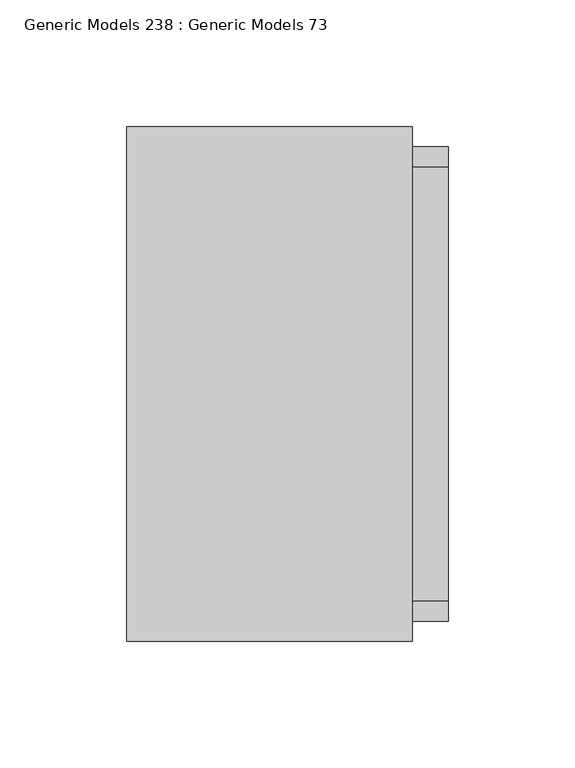
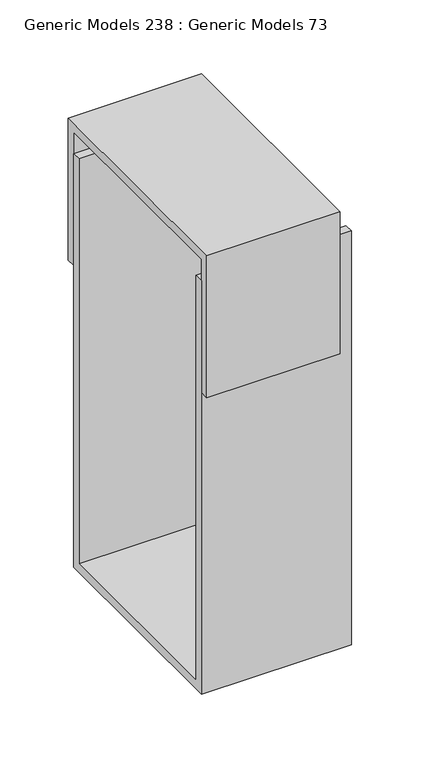
"""IFC4 building model written with IfcOpenShell, lengths in millimetres: proxy geometry, Generic Models 238 : Generic Models 73."""

from ifc_helpers import new_model, si_unit, frame, origin, place, context, project, spatial, polyline, outline, extrude, source, transform, mapped, element, save


def generic_models_238_generic_models_73_f9fcc4d9(model_context):
    return source(origin(), model_context, "Body", "SweptSolid", [
        extrude(outline(polyline([(36501.0832942, 268749.4625), (36313.7582942, 268749.4625), (36313.7582942, 269119.35), (36321.6957942, 269119.35), (36321.6957942, 268757.4), (36493.1457942, 268757.4), (36493.1457942, 269119.35), (36501.0832942, 269119.35), (36501.0832942, 268749.4625)])), frame((31926.2090778, 0.0, 0.0), z_axis=(1.0, 0.0, 0.0), x_axis=(0.0, 1.0, 0.0)), (0.0, 0.0, 1.0), 127.0),
        extrude(outline(polyline([(36509.0207942, 269146.3375), (36509.0207942, 269019.3375), (36501.0832942, 269019.3375), (36501.0832942, 269138.4), (36313.7582942, 269138.4), (36313.7582942, 269019.3375), (36305.8207942, 269019.3375), (36305.8207942, 269146.3375), (36509.0207942, 269146.3375)])), frame((31926.2090778, 0.0, 0.0), z_axis=(1.0, 0.0, 0.0), x_axis=(0.0, 1.0, 0.0)), (0.0, 0.0, 1.0), 112.7125),
    ])


if __name__ == "__main__":
    model = new_model("IFC4")
    model_context = context("Model", 3, world=origin())
    ifc_project = project(units=[si_unit("LENGTHUNIT", "METRE", prefix="MILLI")], contexts=[model_context])
    site = spatial("IfcSite", under=ifc_project)
    building = spatial("IfcBuilding", under=site)
    placement = place(None, origin())
    generic_models_238_generic_models_73_shape = generic_models_238_generic_models_73_f9fcc4d9(model_context)
    element("IfcBuildingElementProxy", 1, Name="Generic Models 238 : Generic Models 73", ObjectType="Generic Models 238 : Generic Models 73", at=placement, inside=building, context=model_context, shape_type="MappedRepresentation", body=[
        mapped(generic_models_238_generic_models_73_shape, transform((0.0, 0.0, 0.0), x_axis=(1.0, 0.0, 0.0), y_axis=(0.0, 1.0, 0.0), z_axis=(0.0, 0.0, 1.0))),
    ])
    save(model, "model.ifc")

# Revit data of these elements
# Element 1 (IfcBuildingElementProxy, "Generic Models 238 : Generic Models 73")
#   Materials on its faces: "5/16 BENT PLATE SADDLE \nW/ 2 1\"DIA. THRU BOLTS"
# Materials
#   "5/16 BENT PLATE SADDLE \nW/ 2 1\"DIA. THRU BOLTS": class "Metal", colour RGB 199 199 199, transparency 0, Description = "Carbon steel", Cost = 0
